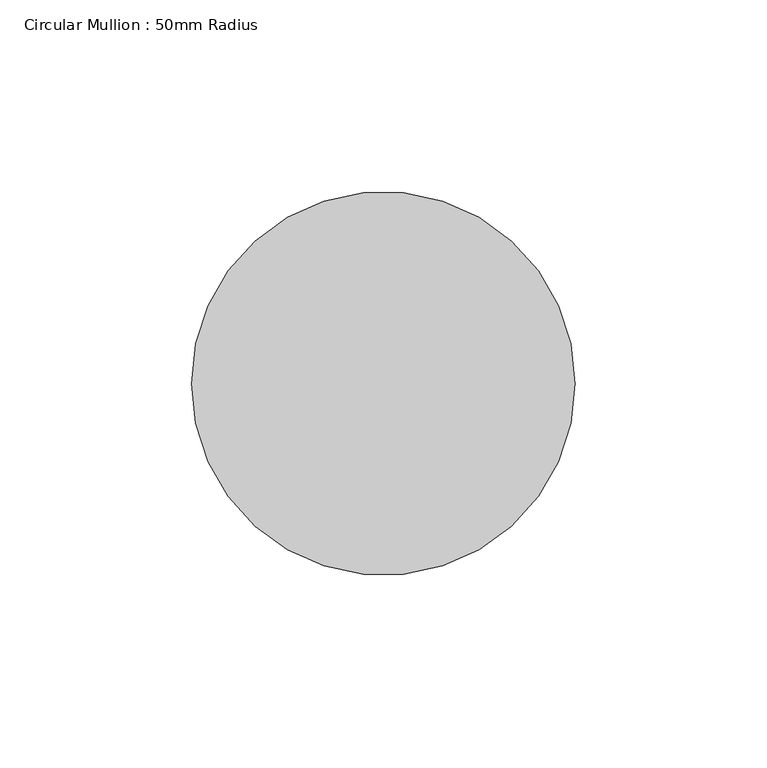
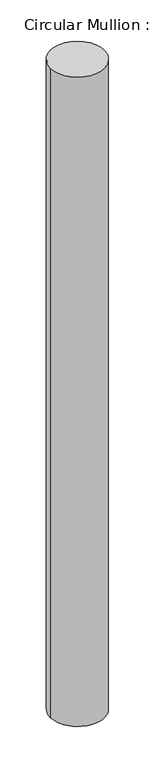
"""IFC4 building model written with IfcOpenShell, lengths in millimetres: member geometry, Circular Mullion : 50mm Radius."""

from ifc_helpers import new_model, si_unit, point, frame, origin, origin_2d, place, context, project, spatial, circle_curve, trimmed, segment, composite_curve, outline, extrude, source, transform, mapped, element, save


def circular_mullion_50mm_radius_b57ce94e(model_context):
    return source(origin(), model_context, "Body", "SweptSolid", [
        extrude(outline(composite_curve([segment(trimmed(circle_curve(origin_2d(), 50.0), [point((50.0, 0.0))], [point((-50.0, 0.0))], False, "CARTESIAN"), True, "CONTINUOUS"), segment(trimmed(circle_curve(origin_2d(), 50.0), [point((-50.0, 0.0))], [point((50.0, 0.0))], False, "CARTESIAN"), True, "CONTINUOUS")], self_intersect=False)), frame((0.0, 0.0, -1273.3492719), z_axis=(0.0, 0.0, 1.0), x_axis=(1.0, 0.0, 0.0)), (0.0, 0.0, 1.0), 1273.3492719),
    ])


if __name__ == "__main__":
    model = new_model("IFC4")
    model_context = context("Model", 3, world=origin())
    ifc_project = project(units=[si_unit("LENGTHUNIT", "METRE", prefix="MILLI")], contexts=[model_context])
    site = spatial("IfcSite", under=ifc_project)
    building = spatial("IfcBuilding", under=site)
    placement = place(None, origin())
    circular_mullion_50mm_radius_shape = circular_mullion_50mm_radius_b57ce94e(model_context)
    element("IfcMember", 1, ObjectType="Circular Mullion : 50mm Radius", at=placement, inside=building, context=model_context, shape_type="MappedRepresentation", body=[
        mapped(circular_mullion_50mm_radius_shape, transform((0.0, 0.0, 0.0), x_axis=(1.0, 0.0, 0.0), y_axis=(0.0, 1.0, 0.0), z_axis=(0.0, 0.0, 1.0))),
    ])
    save(model, "model.ifc")

# Revit data of these elements
# Type "Circular Mullion : 50mm Radius"
#   built-in parameter 1007350 = 0.164042 (stored number, unit not read)
# Element 1 (IfcMember, "Circular Mullion : 50mm Radius")
#   Materials on its faces: "Aluminium"
# Materials
#   "Aluminium": class "Metal", colour RGB 247 247 247, transparency 0, Description = "Aluminium 6061", Cost = 0
